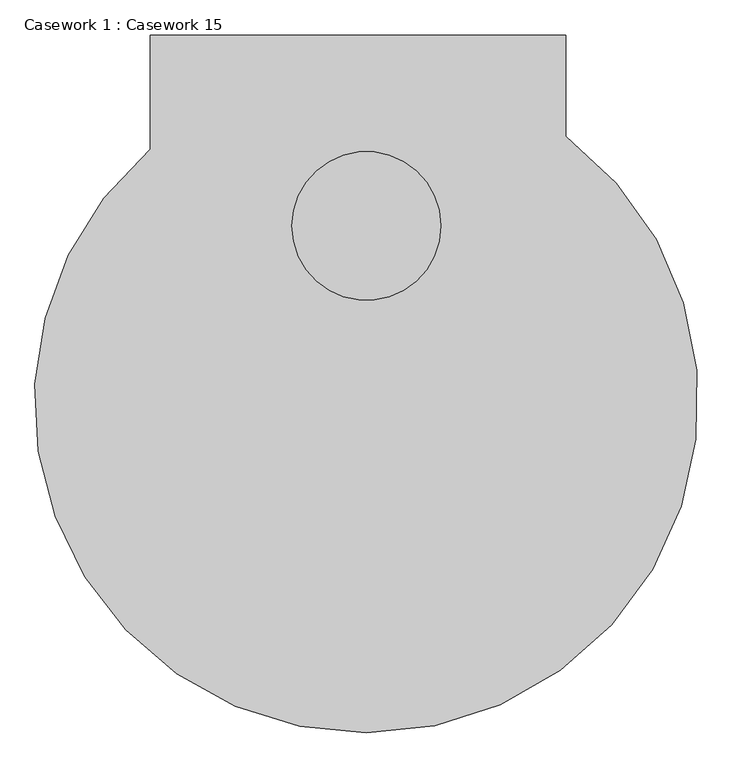
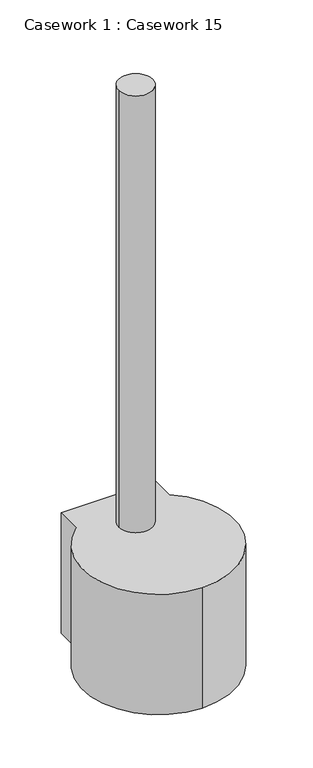
"""IFC4 building model written with IfcOpenShell, lengths in millimetres: furniture geometry, Casework 1 : Casework 15."""

from ifc_helpers import new_model, si_unit, point, frame, frame_2d, origin, origin_with_axes, place, context, project, spatial, polyline, circle_curve, trimmed, segment, composite_curve, outline, extrude, source, transform, mapped, element, save


def casework_1_casework_15_0169ca32(model_context):
    return source(origin(), model_context, "Body", "SweptSolid", [
        extrude(outline(composite_curve([segment(trimmed(circle_curve(frame_2d((-51898.5375322, 254171.2279444)), 203.2), [point((-52101.7375322, 254171.2279444))], [point((-51695.3375322, 254171.2279444))], False, "CARTESIAN"), True, "CONTINUOUS"), segment(trimmed(circle_curve(frame_2d((-51898.5375322, 254171.2279444)), 203.2), [point((-51695.3375322, 254171.2279444))], [point((-52101.7375322, 254171.2279444))], False, "CARTESIAN"), True, "CONTINUOUS")], self_intersect=False)), frame((0.0, 0.0, 1524.0), z_axis=(0.0, 0.0, 1.0), x_axis=(1.0, 0.0, 0.0)), (0.0, 0.0, 1.0), 5532.4382223),
        extrude(outline(composite_curve([segment(polyline([(-52489.2249122, 254693.0154288), (-51353.1783468, 254693.0154288), (-51353.1783468, 254417.5654783)]), True, "CONTINUOUS"), segment(trimmed(circle_curve(frame_2d((-51898.5375322, 253693.585044)), 906.4018482), [point((-51353.1783468, 254417.5654783))], [point((-51898.5375322, 252787.1831958))], False, "CARTESIAN"), True, "CONTINUOUS"), segment(trimmed(circle_curve(frame_2d((-51898.5375322, 253693.585044)), 906.4018482), [point((-51898.5375322, 252787.1831958))], [point((-52489.2249122, 254381.0824836))], False, "CARTESIAN"), True, "CONTINUOUS"), segment(polyline([(-52489.2249122, 254381.0824836), (-52489.2249122, 254693.0154288)]), True, "CONTINUOUS")], self_intersect=False)), origin_with_axes(), (0.0, 0.0, 1.0), 1524.0),
    ])


if __name__ == "__main__":
    model = new_model("IFC4")
    model_context = context("Model", 3, world=origin())
    ifc_project = project(units=[si_unit("LENGTHUNIT", "METRE", prefix="MILLI")], contexts=[model_context])
    site = spatial("IfcSite", under=ifc_project)
    building = spatial("IfcBuilding", under=site)
    placement = place(None, origin())
    casework_1_casework_15_shape = casework_1_casework_15_0169ca32(model_context)
    element("IfcFurniture", 1, ObjectType="Casework 1 : Casework 15", at=placement, inside=building, context=model_context, shape_type="MappedRepresentation", body=[
        mapped(casework_1_casework_15_shape, transform((0.0, 0.0, 0.0), x_axis=(1.0, 0.0, 0.0), y_axis=(0.0, 1.0, 0.0), z_axis=(0.0, 0.0, 1.0))),
    ])
    save(model, "model.ifc")

# Revit data of these elements
# Element 1 (IfcFurniture, "Casework 1 : Casework 15")
#   Materials on its faces: "Dark metal", "ALUMINUM PROFILE AT POLYCARBONATE PANEL"
# Materials
#   "Dark metal": class "Generic", colour RGB 68 68 68, transparency 0, Cost = 0
#   "ALUMINUM PROFILE AT POLYCARBONATE PANEL": class "Metal", colour RGB 244 244 244, transparency 0, Description = "Aluminum 6061", Cost = 0
